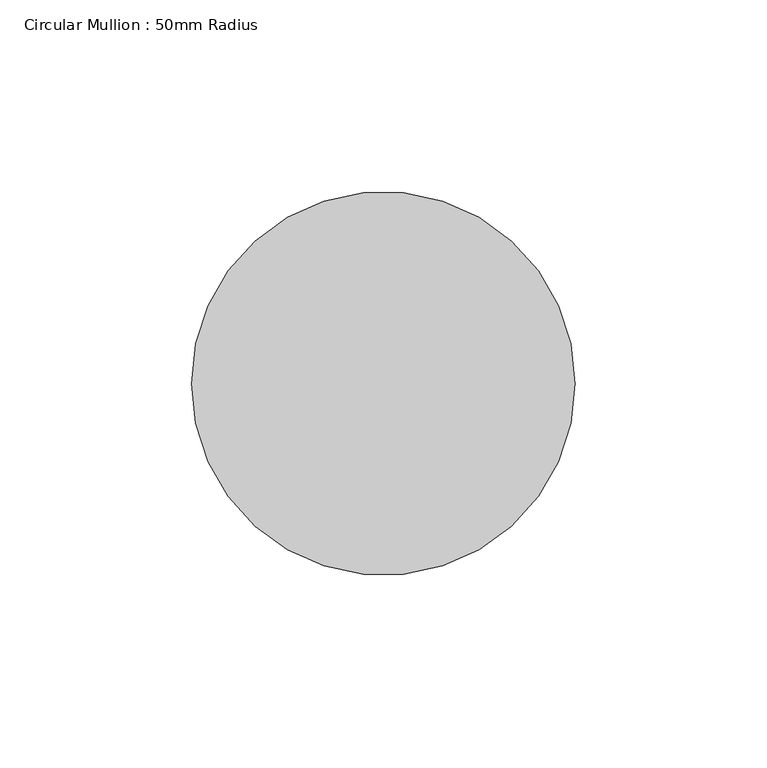
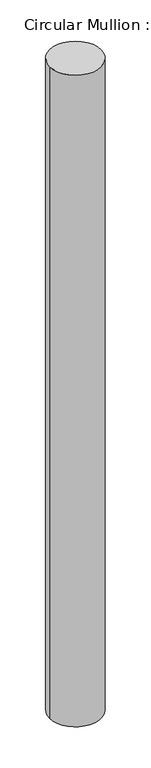
"""IFC4 building model written with IfcOpenShell, lengths in millimetres: member geometry, Circular Mullion : 50mm Radius."""

from ifc_helpers import new_model, si_unit, point, frame, origin, origin_2d, place, context, project, spatial, circle_curve, trimmed, segment, composite_curve, outline, extrude, source, transform, mapped, element, save


def circular_mullion_50mm_radius_2b3d2367(model_context):
    return source(origin(), model_context, "Body", "SweptSolid", [
        extrude(outline(composite_curve([segment(trimmed(circle_curve(origin_2d(), 50.0), [point((50.0, 0.0))], [point((-50.0, 0.0))], False, "CARTESIAN"), True, "CONTINUOUS"), segment(trimmed(circle_curve(origin_2d(), 50.0), [point((-50.0, 0.0))], [point((50.0, 0.0))], False, "CARTESIAN"), True, "CONTINUOUS")], self_intersect=False)), frame((0.0, 0.0, -1336.6641746), z_axis=(0.0, 0.0, 1.0), x_axis=(1.0, 0.0, 0.0)), (0.0, 0.0, 1.0), 1336.6641746),
    ])


if __name__ == "__main__":
    model = new_model("IFC4")
    model_context = context("Model", 3, world=origin())
    ifc_project = project(units=[si_unit("LENGTHUNIT", "METRE", prefix="MILLI")], contexts=[model_context])
    site = spatial("IfcSite", under=ifc_project)
    building = spatial("IfcBuilding", under=site)
    placement = place(None, origin())
    circular_mullion_50mm_radius_shape = circular_mullion_50mm_radius_2b3d2367(model_context)
    element("IfcMember", 1, ObjectType="Circular Mullion : 50mm Radius", at=placement, inside=building, context=model_context, shape_type="MappedRepresentation", body=[
        mapped(circular_mullion_50mm_radius_shape, transform((0.0, 0.0, 0.0), x_axis=(1.0, 0.0, 0.0), y_axis=(0.0, 1.0, 0.0), z_axis=(0.0, 0.0, 1.0))),
    ])
    save(model, "model.ifc")

# Revit data of these elements
# Type "Circular Mullion : 50mm Radius"
#   built-in parameter 1007350 = 0.164042 (stored number, unit not read)
# Element 1 (IfcMember, "Circular Mullion : 50mm Radius")
#   Materials on its faces: "Aluminium"
# Materials
#   "Aluminium": class "Metal", colour RGB 247 247 247, transparency 0, Description = "Aluminium 6061", Cost = 0
